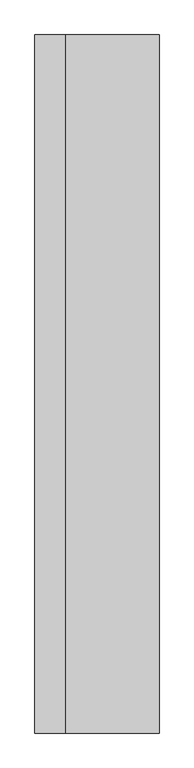
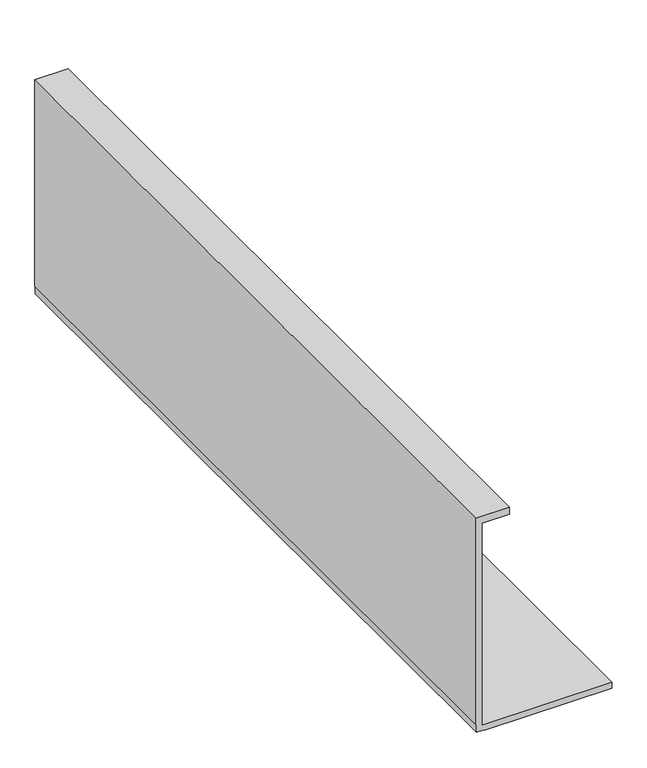
"""IFC4 building model written with IfcOpenShell, lengths in millimetres: proxy geometry, Gypsum023 17893 : Gypsum023 17893."""

from ifc_helpers import new_model, si_unit, frame, origin, place, context, project, spatial, polyline, outline, extrude, source, transform, mapped, element, save


def generic_models_781c0796(model_context):
    return source(origin(), model_context, "Body", "SweptSolid", [
        extrude(outline(polyline([(39557.071, 7559.210084), (39572.946, 7559.210084), (39572.946, 7218.5762049), (40131.746, 7218.5762049), (40131.746, 7290.9824219), (40150.796, 7290.9824219), (40150.796, 7203.5713569), (39579.5041839, 7203.5713569), (39579.5041839, 7204.8513569), (39558.351, 7204.8513569), (39558.351, 7226.0045408), (39557.071, 7226.0045408), (39557.071, 7559.210084)])), frame((0.0, -3747.9491938, 0.0), z_axis=(0.0, 1.0, 0.0), x_axis=(0.0, 0.0, 1.0)), (0.0, 0.0, 1.0), 1999.85),
    ])


if __name__ == "__main__":
    model = new_model("IFC4")
    model_context = context("Model", 3, world=origin())
    ifc_project = project(units=[si_unit("LENGTHUNIT", "METRE", prefix="MILLI")], contexts=[model_context])
    site = spatial("IfcSite", under=ifc_project)
    building = spatial("IfcBuilding", under=site)
    placement = place(None, origin())
    generic_models_shape = generic_models_781c0796(model_context)
    element("IfcBuildingElementProxy", 1, Name="Gypsum023 17893 : Gypsum023 17893", ObjectType="Gypsum023 17893 : Gypsum023 17893", at=placement, inside=building, context=model_context, shape_type="MappedRepresentation", body=[
        mapped(generic_models_shape, transform((0.0, 0.0, 0.0), x_axis=(1.0, 0.0, 0.0), y_axis=(0.0, 1.0, 0.0), z_axis=(0.0, 0.0, 1.0))),
    ])
    save(model, "model.ifc")

# Revit data of these elements
# Type "Gypsum023 17893 : Gypsum023 17893"
#   NameOverride = "Gypsum023"
# Element 1 (IfcBuildingElementProxy, "Gypsum023 17893 : Gypsum023 17893")
#   Materials on its faces: "5/8\" GYPSUM BOARD"
# Materials
#   "5/8\" GYPSUM BOARD": class "Unassigned", colour RGB 214 214 214, transparency 0, Cost = 0
